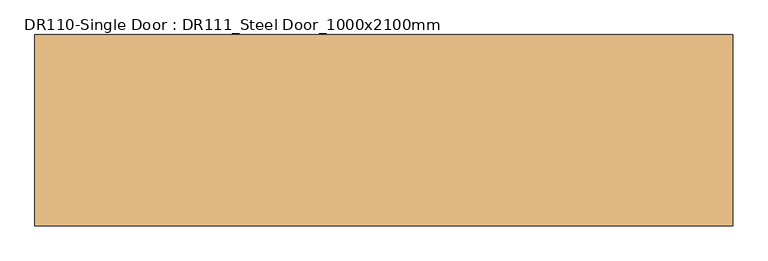
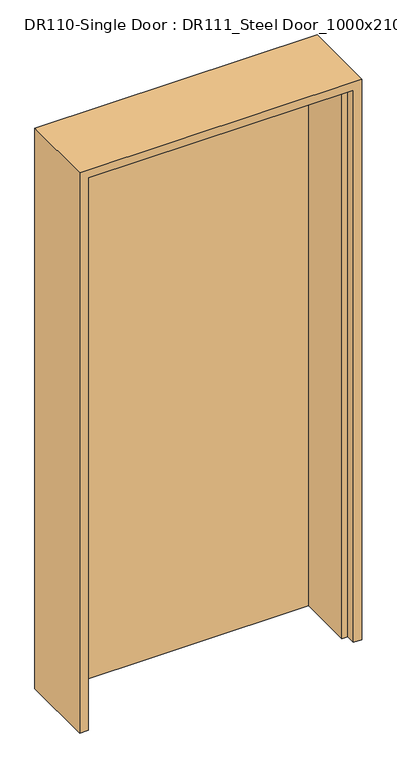
"""IFC4 building model written with IfcOpenShell, lengths in millimetres: door geometry, DR110-Single Door : DR111_Steel Door_1000x2100mm."""

from ifc_helpers import new_model, si_unit, origin, origin_with_axes, place, context, project, spatial, polyline, outline, extrude, faceted_brep, source, transform, mapped, element, save


def dr110_single_door_dr111_steel_door_1000x2100mm_d0b51d4b(model_context):
    return source(origin(), model_context, "Body", "SolidModel", [
        extrude(outline(polyline([(470.0, 137.0), (470.0, 102.0), (-470.0, 102.0), (-470.0, 137.0), (470.0, 137.0)])), origin_with_axes(), (0.0, 0.0, 1.0), 2070.0),
        faceted_brep([(470.0, 137.0, 0.0), (500.0, 137.0, 0.0), (500.0, -137.0, 0.0), (470.0, -137.0, 0.0), (470.0, -102.0, 0.0), (450.0, -102.0, 0.0), (450.0, 102.0, 0.0), (470.0, 102.0, 0.0), (470.0, 137.0, 2070.0), (-470.0, 137.0, 2070.0), (-470.0, 137.0, 0.0), (-500.0, 137.0, 0.0), (-500.0, 137.0, 2100.0), (500.0, 137.0, 2100.0), (500.0, -137.0, 2100.0), (-500.0, -137.0, 2100.0), (-500.0, -137.0, 0.0), (-470.0, -137.0, 0.0), (-470.0, -137.0, 2070.0), (470.0, -137.0, 2070.0), (470.0, -102.0, 2070.0), (-470.0, -102.0, 2070.0), (-470.0, -102.0, 0.0), (-450.0, -102.0, 0.0), (-450.0, -102.0, 2050.0), (450.0, -102.0, 2050.0), (450.0, 102.0, 2050.0), (-450.0, 102.0, 2050.0), (-450.0, 102.0, 0.0), (-470.0, 102.0, 0.0), (-470.0, 102.0, 2070.0), (470.0, 102.0, 2070.0)], [[[0, 1, 2, 3, 4, 5, 6, 7]], [[1, 0, 8, 9, 10, 11, 12, 13]], [[2, 1, 13, 14]], [[3, 2, 14, 15, 16, 17, 18, 19]], [[4, 3, 19, 20]], [[5, 4, 20, 21, 22, 23, 24, 25]], [[6, 5, 25, 26]], [[7, 6, 26, 27, 28, 29, 30, 31]], [[0, 7, 31, 8]], [[9, 30, 29, 10]], [[10, 29, 28, 23, 22, 17, 16, 11]], [[15, 12, 11, 16]], [[21, 18, 17, 22]], [[27, 24, 23, 28]], [[14, 13, 12, 15]], [[20, 19, 18, 21]], [[26, 25, 24, 27]], [[8, 31, 30, 9]]]),
    ])


if __name__ == "__main__":
    model = new_model("IFC4")
    model_context = context("Model", 3, world=origin())
    ifc_project = project(units=[si_unit("LENGTHUNIT", "METRE", prefix="MILLI")], contexts=[model_context])
    site = spatial("IfcSite", under=ifc_project)
    building = spatial("IfcBuilding", under=site)
    placement = place(None, origin())
    dr110_single_door_dr111_steel_door_1000x2100mm_shape = dr110_single_door_dr111_steel_door_1000x2100mm_d0b51d4b(model_context)
    element("IfcDoor", 1, ObjectType="DR110-Single Door : DR111_Steel Door_1000x2100mm", at=placement, inside=building, context=model_context, shape_type="MappedRepresentation", body=[
        mapped(dr110_single_door_dr111_steel_door_1000x2100mm_shape, transform((0.0, 0.0, 0.0), x_axis=(1.0, 0.0, 0.0), y_axis=(0.0, 1.0, 0.0), z_axis=(0.0, 0.0, 1.0))),
    ])
    save(model, "model.ifc")

# Revit data of these elements
# Type "DR110-Single Door : DR111_Steel Door_1000x2100mm"
#   Type Mark = "SD"
#   Analytic Construction = "<None>"
#   프레임 투영 외부. = 25 mm
#   프레임 투영 내부. = 25 mm
#   프레임 폭 = 75 mm
#   Height = 2100 mm
#   Width = 1000 mm
#   Define Thermal Properties by = 1
#   문 패널 = SD1 문 패널
#   문 프레임 = A04AQ098-00002_Steel Door_non FP_single
#   Function = (empty or 0)
#   Wall Closure = (empty or 0)
# Element 1 (IfcDoor, "DR110-Single Door : DR111_Steel Door_1000x2100mm")
#   Materials on its faces: "A04AQ098-00002_Steel Door_non FP_single", "SD1 문 패널"
# Materials
#   "SD1 문 패널": class "금속", colour RGB 247 247 247, transparency 0, Description = "STEEL DOOR (1000Wx2100H)"
#   "A04AQ098-00002_Steel Door_non FP_single": class "금속", colour RGB 247 247 247, transparency 0, Description = "Steel Door", W00) Work Master Code = "A04AQ098-00002", W01) Work Master_Lv1 = "Finishing Work", W02) Work Master_Lv2 = "Door & Window Work", W03) Work Master_Spec.1 = "Steel Door w/ Steel Frame", W04) Work Master_Spec.2 = "Fire Protective Rating: N/A, Single Door", W05) Work Master_Spec.3 = "w/ Hardware & Accessories", Cost = 0
